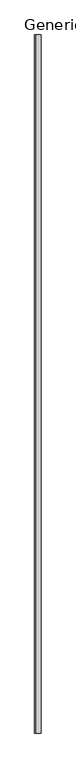
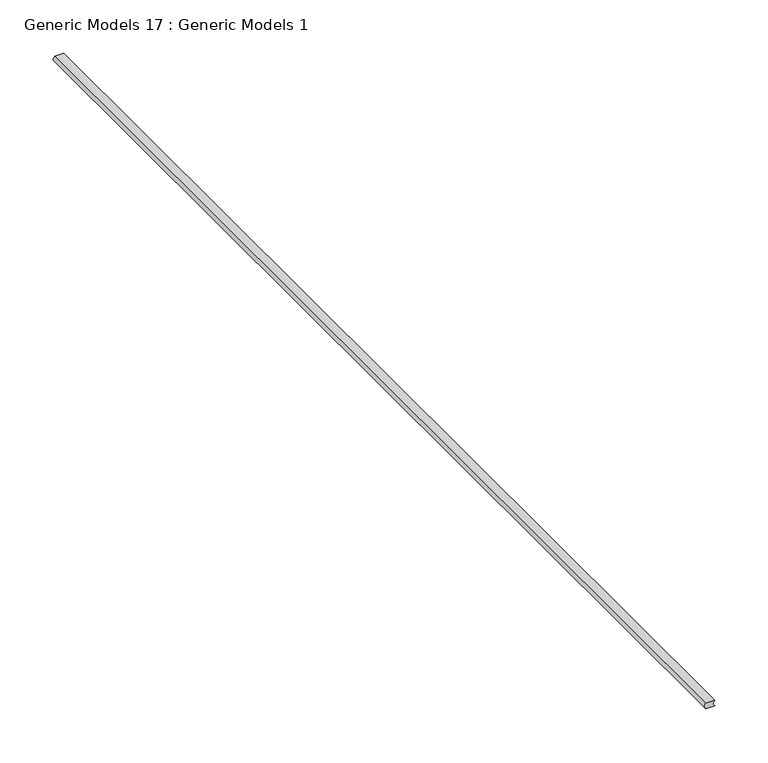
"""IFC4 building model written with IfcOpenShell, lengths in millimetres: proxy geometry, Generic Models 17 : Generic Models 1."""

import ifcopenshell
import ifcopenshell.guid

model = None  # the IFC model being written
_history = None  # IfcOwnerHistory: only IFC2X3 demands one
_inside = {}  # id of a spatial element -> (the spatial element, [elements in it])
_under = {}  # id of a project, library or spatial element -> (it, [spatial elements below it])
_declared = {}  # id of a project -> (the project, [libraries it declares])
_typed = {}  # id of a type object -> (the type object, [elements of that type])
_made_of = {}  # id of a material, layer set ... -> (it, [elements and type objects made of it])


def new_model(schema):
    """Start an empty IFC model of exactly this schema.

    Asked for "IFC4X3", IfcOpenShell would pick the latest addendum, in which some entities
    have other attributes; the version numbers below select the first issue.
    IFC2X3 requires an IfcOwnerHistory on every rooted entity: one is made here for all.
    """
    global model, _history
    if schema == "IFC4X3":
        model = ifcopenshell.file(schema_version=(4, 3, 0, 0))
    else:
        model = ifcopenshell.file(schema=schema)
    _inside.clear()
    _under.clear()
    _declared.clear()
    _typed.clear()
    _made_of.clear()
    _history = None
    if model.schema == "IFC2X3":
        org = make("IfcOrganization", Name="unknown")
        user = make(
            "IfcPersonAndOrganization",
            ThePerson=make("IfcPerson", FamilyName="unknown"),
            TheOrganization=org,
        )
        app = make(
            "IfcApplication",
            ApplicationDeveloper=org,
            Version="unknown",
            ApplicationFullName="unknown",
            ApplicationIdentifier="unknown",
        )
        _history = make(
            "IfcOwnerHistory",
            OwningUser=user,
            OwningApplication=app,
            ChangeAction="ADDED",
            CreationDate=0,
        )
    return model


def make(cls, **values):
    """One entity of the class cls with the attributes given. An attribute that is None is left unset."""
    return model.create_entity(
        cls, **{name: value for name, value in values.items() if value is not None}
    )


def rooted(cls, **values):
    """An entity with a GlobalId (a new one), such as an element, a storey or a relation."""
    return make(cls, GlobalId=ifcopenshell.guid.new(), OwnerHistory=_history, **values)


def si_unit(unit_type, name, prefix=None):
    """IfcSIUnit, for example si_unit("LENGTHUNIT", "METRE", prefix="MILLI")."""
    return make("IfcSIUnit", UnitType=unit_type, Prefix=prefix, Name=name)


def assignment(units):
    """IfcUnitAssignment: the units of a project."""
    return None if units is None else make("IfcUnitAssignment", Units=units)


def point(xyz):
    """IfcCartesianPoint."""
    return None if xyz is None else make("IfcCartesianPoint", Coordinates=xyz)


def direction(xyz):
    """IfcDirection."""
    return None if xyz is None else make("IfcDirection", DirectionRatios=xyz)


def frame(location, z_axis=None, x_axis=None):
    """IfcAxis2Placement3D, a coordinate frame: its origin and axes. An axis left out is left unset."""
    return make(
        "IfcAxis2Placement3D",
        Location=point(location),
        Axis=direction(z_axis),
        RefDirection=direction(x_axis),
    )


def frame_2d(location, x_axis=None):
    """IfcAxis2Placement2D, a coordinate frame in the plane: its origin and x axis."""
    return make(
        "IfcAxis2Placement2D", Location=point(location), RefDirection=direction(x_axis)
    )


def origin():
    """The frame at (0, 0, 0) with its axes left unset."""
    return frame((0.0, 0.0, 0.0))


def place(relative_to, where):
    """IfcLocalPlacement: puts the frame where relative to a parent placement (None: the world)."""
    return make(
        "IfcLocalPlacement", PlacementRelTo=relative_to, RelativePlacement=where
    )


def context(
    kind, dimensions, precision=None, world=None, true_north=None, identifier=None
):
    """IfcGeometricRepresentationContext, for example the 3D "Model" context."""
    return make(
        "IfcGeometricRepresentationContext",
        ContextIdentifier=identifier,
        ContextType=kind,
        CoordinateSpaceDimension=dimensions,
        Precision=precision,
        WorldCoordinateSystem=world,
        TrueNorth=true_north,
    )


def project(units=None, contexts=None):
    """IfcProject with its units and contexts."""
    return rooted(
        "IfcProject",
        Name="project",
        RepresentationContexts=contexts,
        UnitsInContext=assignment(units),
    )


def spatial(cls, under=None, at=None, **own):
    """A site, building, storey or space (cls), placed at a placement, below another one or the project."""
    s = rooted(cls, ObjectPlacement=at, **own)
    if under is not None:
        _under.setdefault(under.id(), (under, []))[1].append(s)
    return s


def polyline(points):
    """IfcPolyline through the points."""
    return make("IfcPolyline", Points=[point(p) for p in points])


def circle_curve(where, radius):
    """IfcCircle in the frame where."""
    return make("IfcCircle", Position=where, Radius=radius)


def trimmed(basis, trim1, trim2, sense, master):
    """IfcTrimmedCurve: the piece of a basis curve between two trims."""
    return make(
        "IfcTrimmedCurve",
        BasisCurve=basis,
        Trim1=trim1,
        Trim2=trim2,
        SenseAgreement=sense,
        MasterRepresentation=master,
    )


def segment(curve, same_sense, transition):
    """IfcCompositeCurveSegment."""
    return make(
        "IfcCompositeCurveSegment",
        Transition=transition,
        SameSense=same_sense,
        ParentCurve=curve,
    )


def composite_curve(segments, self_intersect=None):
    """IfcCompositeCurve: segments joined end to end."""
    return make("IfcCompositeCurve", Segments=segments, SelfIntersect=self_intersect)


def outline(outer, holes=None, kind="AREA"):
    """IfcArbitraryClosedProfileDef: a profile drawn as a closed curve; with holes, ...WithVoids."""
    if holes is None:
        return make("IfcArbitraryClosedProfileDef", ProfileType=kind, OuterCurve=outer)
    return make(
        "IfcArbitraryProfileDefWithVoids",
        ProfileType=kind,
        OuterCurve=outer,
        InnerCurves=holes,
    )


def extrude(swept, where, along, depth):
    """IfcExtrudedAreaSolid: the profile swept, set in the frame where, extruded along a direction by depth."""
    return make(
        "IfcExtrudedAreaSolid",
        SweptArea=swept,
        Position=where,
        ExtrudedDirection=direction(along),
        Depth=depth,
    )


def shape(context_of_items, identifier, shape_type, items):
    """IfcShapeRepresentation: the items that make up one representation, for example the "Body"."""
    return make(
        "IfcShapeRepresentation",
        ContextOfItems=context_of_items,
        RepresentationIdentifier=identifier,
        RepresentationType=shape_type,
        Items=items,
    )


def source(mapping_origin, context_of_items, identifier, shape_type, items):
    """IfcRepresentationMap: a shape defined once, which mapped items show again and again."""
    return make(
        "IfcRepresentationMap",
        MappingOrigin=mapping_origin,
        MappedRepresentation=shape(context_of_items, identifier, shape_type, items),
    )


def transform(
    local_origin,
    x_axis=None,
    y_axis=None,
    z_axis=None,
    scale=None,
    scale2=None,
    scale3=None,
    uniform=True,
):
    """IfcCartesianTransformationOperator3D, or its non-uniform kind. x_axis, y_axis, z_axis: its Axis1, 2, 3."""
    if uniform:
        return make(
            "IfcCartesianTransformationOperator3D",
            Axis1=direction(x_axis),
            Axis2=direction(y_axis),
            LocalOrigin=point(local_origin),
            Scale=scale,
            Axis3=direction(z_axis),
        )
    return make(
        "IfcCartesianTransformationOperator3DnonUniform",
        Axis1=direction(x_axis),
        Axis2=direction(y_axis),
        LocalOrigin=point(local_origin),
        Scale=scale,
        Axis3=direction(z_axis),
        Scale2=scale2,
        Scale3=scale3,
    )


def mapped(mapping_source, mapping_target):
    """IfcMappedItem: shows the shape of a source again, moved by a transform."""
    return make(
        "IfcMappedItem", MappingSource=mapping_source, MappingTarget=mapping_target
    )


def made_of(thing, what):
    """Note that an element or type object is made of a material, layer set ...; save() writes the relation."""
    if what is not None:
        _made_of.setdefault(what.id(), (what, []))[1].append(thing)
    return thing


def element(
    cls,
    number,
    at=None,
    inside=None,
    cuts=None,
    type_object=None,
    material=None,
    context=None,
    identifier="Body",
    shape_type=None,
    held_by="IfcProductDefinitionShape",
    body=None,
    shapes=None,
    **own,
):
    """One element of the class cls, such as IfcWall. Its Tag is "e" and its number.

    at: its placement. inside: the storey or other place that contains it. cuts: it is an
    opening in that element (IfcRelVoidsElement). A single representation is given by context,
    identifier, shape_type and body (its items); several are given by shapes. held_by: the class
    of the entity that holds the representations. save() writes the other relations.
    """
    e = rooted(cls, Tag="e%d" % number, ObjectPlacement=at, **own)
    if body is not None:
        shapes = [shape(context, identifier, shape_type, body)]
    if shapes is not None:
        e.Representation = make(held_by, Representations=shapes)
    if inside is not None:
        _inside.setdefault(inside.id(), (inside, []))[1].append(e)
    if cuts is not None:
        rooted(
            "IfcRelVoidsElement", RelatingBuildingElement=cuts, RelatedOpeningElement=e
        )
    if type_object is not None:
        _typed.setdefault(type_object.id(), (type_object, []))[1].append(e)
    return made_of(e, material)


def aggregate(whole, parts):
    """IfcRelAggregates: a whole, such as a stair, and the parts it consists of."""
    return rooted("IfcRelAggregates", RelatingObject=whole, RelatedObjects=parts)


def save(model, path):
    """Write the relations noted so far, then the file.

    IfcRelAggregates (storeys below a building ...), IfcRelContainedInSpatialStructure (elements
    in a storey), IfcRelDefinesByType, IfcRelAssociatesMaterial and IfcRelDeclares: one each for
    every whole, place, type object, material and project.
    """
    for whole, parts in _under.values():
        aggregate(whole, parts)
    for where, things in _inside.values():
        rooted(
            "IfcRelContainedInSpatialStructure",
            RelatedElements=things,
            RelatingStructure=where,
        )
    for kind, things in _typed.values():
        rooted("IfcRelDefinesByType", RelatedObjects=things, RelatingType=kind)
    for what, things in _made_of.values():
        rooted("IfcRelAssociatesMaterial", RelatedObjects=things, RelatingMaterial=what)
    for by, libraries in _declared.values():
        rooted("IfcRelDeclares", RelatingContext=by, RelatedDefinitions=libraries)
    model.write(path)


def generic_models_17_generic_models_1_4289aad1(model_context):
    return source(origin(), model_context, "Body", "SweptSolid", [
        extrude(outline(composite_curve([segment(trimmed(circle_curve(frame_2d((3.175, 51021.9897405)), 4.3100275), [point((0.0, 51019.075))], [point((6.35, 51019.075))], True, "CARTESIAN"), True, "CONTINUOUS"), segment(polyline([(6.35, 51019.075), (6.35, 51009.55)]), True, "CONTINUOUS"), segment(trimmed(circle_curve(frame_2d((3.175, 51012.4647405)), 4.3100275), [point((6.35, 51009.55))], [point((0.0, 51009.55))], False, "CARTESIAN"), True, "CONTINUOUS"), segment(polyline([(0.0, 51009.55), (0.0, 51019.075)]), True, "CONTINUOUS")], self_intersect=False)), frame((0.0, 0.0, 0.0), z_axis=(0.0, 1.0, 0.0), x_axis=(0.0, 0.0, 1.0)), (0.0, 0.0, 1.0), 1219.2),
    ])


if __name__ == "__main__":
    model = new_model("IFC4")
    model_context = context("Model", 3, world=origin())
    ifc_project = project(units=[si_unit("LENGTHUNIT", "METRE", prefix="MILLI")], contexts=[model_context])
    site = spatial("IfcSite", under=ifc_project)
    building = spatial("IfcBuilding", under=site)
    placement = place(None, origin())
    generic_models_17_generic_models_1_shape = generic_models_17_generic_models_1_4289aad1(model_context)
    element("IfcBuildingElementProxy", 1, Name="Generic Models 17 : Generic Models 1", ObjectType="Generic Models 17 : Generic Models 1", at=placement, inside=building, context=model_context, shape_type="MappedRepresentation", body=[
        mapped(generic_models_17_generic_models_1_shape, transform((0.0, 0.0, 0.0), x_axis=(1.0, 0.0, 0.0), y_axis=(0.0, 1.0, 0.0), z_axis=(0.0, 0.0, 1.0))),
    ])
    save(model, "model.ifc")

# Revit data of these elements
# Element 1 (IfcBuildingElementProxy, "Generic Models 17 : Generic Models 1")
#   Materials on its faces: "ACOUSTICAL SEALANT"
# Materials
#   "ACOUSTICAL SEALANT": class "Unassigned", colour RGB 120 120 120, transparency 0, Cost = 0
